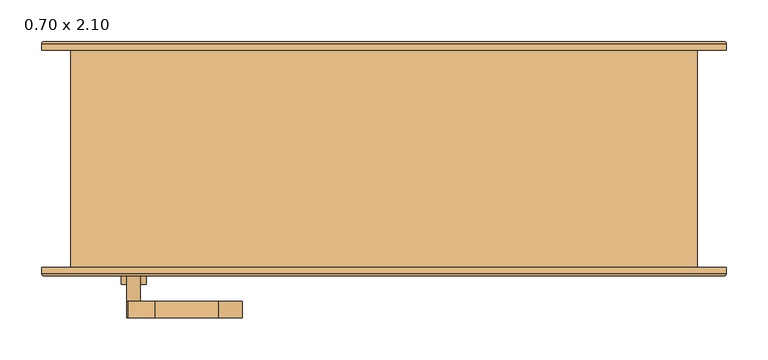
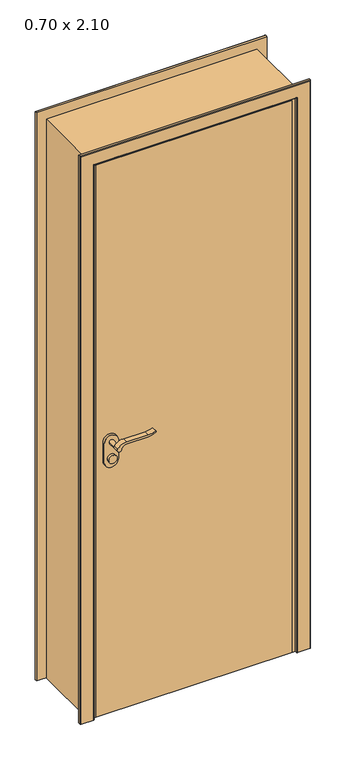
"""IFC4 building model written with IfcOpenShell, lengths in millimetres: door geometry, .CC_ND 300_PORTA SIMPLES DE ABRIR_COM EXTENSÃO : 0.70 x 2.10."""

from ifc_helpers import new_model, si_unit, point, frame, frame_2d, origin, origin_with_axes, place, context, project, spatial, polyline, circle_curve, ellipse_curve, trimmed, segment, composite_curve, outline, extrude, faceted_brep, source, transform, mapped, element, save
from ifc_brep_helpers import plane_surface, cylinder_surface, advanced_brep


def door_0_70_x_2_10_365ff999(model_context):
    return source(origin(), model_context, "Body", "SolidModel", [
        extrude(outline(composite_curve([segment(trimmed(circle_curve(frame_2d((964.5, -300.0)), 15.0), [point((964.5, -285.0))], [point((964.5, -315.0))], False, "CARTESIAN"), True, "CONTINUOUS"), segment(trimmed(circle_curve(frame_2d((964.5, -300.0)), 15.0), [point((964.5, -315.0))], [point((964.5, -285.0))], False, "CARTESIAN"), True, "CONTINUOUS")], self_intersect=False)), frame((0.0, -163.0, 0.0), z_axis=(0.0, 1.0, 0.0), x_axis=(0.0, 0.0, 1.0)), (0.0, 0.0, 1.0), 10.0),
        extrude(outline(composite_curve([segment(trimmed(circle_curve(frame_2d((964.5, -300.0)), 15.0), [point((964.5, -285.0))], [point((964.5, -315.0))], False, "CARTESIAN"), True, "CONTINUOUS"), segment(trimmed(circle_curve(frame_2d((964.5, -300.0)), 15.0), [point((964.5, -315.0))], [point((964.5, -285.0))], False, "CARTESIAN"), True, "CONTINUOUS")], self_intersect=False)), frame((0.0, -103.0, 0.0), z_axis=(0.0, 1.0, 0.0), x_axis=(0.0, 0.0, 1.0)), (0.0, 0.0, 1.0), 10.0),
        extrude(outline(composite_curve([segment(trimmed(circle_curve(frame_2d((1024.5, -300.0)), 8.0), [point((1029.1523287, -306.5081363))], [point((1024.5, -292.0))], False, "CARTESIAN"), True, "CONTINUOUS"), segment(trimmed(circle_curve(frame_2d((1019.3738613, -274.6138099)), 18.1261387), [point((1024.5, -292.0))], [point((1037.5, -274.6138099))], True, "CARTESIAN"), True, "CONTINUOUS"), segment(polyline([(1037.5, -274.6138099), (1037.5, -198.3564091)]), True, "CONTINUOUS"), segment(trimmed(circle_curve(frame_2d((1096.7709207, -201.9396612)), 59.3791355), [point((1037.5, -198.3564091))], [point((1046.7135558, -170.0))], False, "CARTESIAN"), True, "CONTINUOUS"), segment(polyline([(1046.7135558, -170.0), (1049.5, -170.0)]), True, "CONTINUOUS"), segment(trimmed(circle_curve(frame_2d((1127.7850638, -198.4227909)), 83.2850902), [point((1049.5, -170.0))], [point((1044.5, -198.3564091))], True, "CARTESIAN"), True, "CONTINUOUS"), segment(polyline([(1044.5, -198.3564091), (1044.5, -274.6325667)]), True, "CONTINUOUS"), segment(trimmed(circle_curve(frame_2d((1007.2555521, -276.3324871)), 37.2832219), [point((1044.5, -274.6325667))], [point((1029.1523287, -306.5081363))], False, "CARTESIAN"), True, "CONTINUOUS")], self_intersect=False)), frame((0.0, -203.0, 0.0), z_axis=(0.0, 1.0, 0.0), x_axis=(0.0, 0.0, 1.0)), (0.0, 0.0, 1.0), 20.0),
        extrude(outline(composite_curve([segment(trimmed(circle_curve(frame_2d((1019.3738682, -274.6138122)), 18.1261318), [point((1024.4999903, -292.0))], [point((1037.5, -274.6138122))], True, "CARTESIAN"), True, "CONTINUOUS"), segment(polyline([(1037.5, -274.6138122), (1037.5, -198.3564091)]), True, "CONTINUOUS"), segment(trimmed(circle_curve(frame_2d((1096.7709207, -201.9396612)), 59.3791355), [point((1037.5, -198.3564091))], [point((1046.7135558, -170.0))], False, "CARTESIAN"), True, "CONTINUOUS"), segment(polyline([(1046.7135558, -170.0), (1049.5, -170.0)]), True, "CONTINUOUS"), segment(trimmed(circle_curve(frame_2d((1127.7850638, -198.4227909)), 83.2850902), [point((1049.5, -170.0))], [point((1044.5, -198.3564091))], True, "CARTESIAN"), True, "CONTINUOUS"), segment(polyline([(1044.5, -198.3564091), (1044.5, -274.6325667)]), True, "CONTINUOUS"), segment(trimmed(circle_curve(frame_2d((1007.2555521, -276.3324871)), 37.2832219), [point((1044.5, -274.6325667))], [point((1029.1523287, -306.5081363))], False, "CARTESIAN"), True, "CONTINUOUS"), segment(trimmed(circle_curve(frame_2d((1024.5, -300.0)), 8.0), [point((1029.1523287, -306.5081363))], [point((1024.4999903, -292.0))], False, "CARTESIAN"), True, "CONTINUOUS")], self_intersect=False)), frame((0.0, -73.0, 0.0), z_axis=(0.0, 1.0, 0.0), x_axis=(0.0, 0.0, 1.0)), (0.0, 0.0, 1.0), 20.0),
        extrude(outline(composite_curve([segment(trimmed(circle_curve(frame_2d((1024.5, -300.0)), 8.0), [point((1024.5, -292.0))], [point((1024.5, -308.0))], False, "CARTESIAN"), True, "CONTINUOUS"), segment(trimmed(circle_curve(frame_2d((1024.5, -300.0)), 8.0), [point((1024.5, -308.0))], [point((1024.5, -292.0))], False, "CARTESIAN"), True, "CONTINUOUS")], self_intersect=False)), frame((0.0, -183.0, 0.0), z_axis=(0.0, 1.0, 0.0), x_axis=(0.0, 0.0, 1.0)), (0.0, 0.0, 1.0), 30.0),
        extrude(outline(composite_curve([segment(trimmed(circle_curve(frame_2d((1024.5, -300.0)), 8.0), [point((1024.5, -292.0))], [point((1024.5, -308.0))], False, "CARTESIAN"), True, "CONTINUOUS"), segment(trimmed(circle_curve(frame_2d((1024.5, -300.0)), 8.0), [point((1024.5, -308.0))], [point((1024.5, -292.0))], False, "CARTESIAN"), True, "CONTINUOUS")], self_intersect=False)), frame((0.0, -103.0, 0.0), z_axis=(0.0, 1.0, 0.0), x_axis=(0.0, 0.0, 1.0)), (0.0, 0.0, 1.0), 30.0),
        extrude(outline(composite_curve([segment(trimmed(circle_curve(frame_2d((954.5, -300.0)), 25.0), [point((954.5, -325.0))], [point((954.5, -275.0))], False, "CARTESIAN"), True, "CONTINUOUS"), segment(polyline([(954.5, -275.0), (1024.5, -275.0)]), True, "CONTINUOUS"), segment(trimmed(circle_curve(frame_2d((1024.5, -300.0)), 25.0), [point((1024.5, -275.0))], [point((1024.5, -325.0))], False, "CARTESIAN"), True, "CONTINUOUS"), segment(polyline([(1024.5, -325.0), (954.5, -325.0)]), True, "CONTINUOUS")], self_intersect=False)), frame((0.0, -153.0, 0.0), z_axis=(0.0, 1.0, 0.0), x_axis=(0.0, 0.0, 1.0)), (0.0, 0.0, 1.0), 10.0),
        extrude(outline(composite_curve([segment(trimmed(circle_curve(frame_2d((954.5, -300.0)), 25.0), [point((954.5, -325.0))], [point((954.5, -275.0))], False, "CARTESIAN"), True, "CONTINUOUS"), segment(polyline([(954.5, -275.0), (1024.5, -275.0)]), True, "CONTINUOUS"), segment(trimmed(circle_curve(frame_2d((1024.5, -300.0)), 25.0), [point((1024.5, -275.0))], [point((1024.5, -325.0))], False, "CARTESIAN"), True, "CONTINUOUS"), segment(polyline([(1024.5, -325.0), (954.5, -325.0)]), True, "CONTINUOUS")], self_intersect=False)), frame((0.0, -113.0, 0.0), z_axis=(0.0, 1.0, 0.0), x_axis=(0.0, 0.0, 1.0)), (0.0, 0.0, 1.0), 10.0),
        advanced_brep(
        [(-410.0, -143.0, 0.0), (-360.0, -143.0, 0.0), (-360.0, -150.0, 0.0), (-363.0, -153.0, 0.0), (-407.0, -153.0, 0.0), (-410.0, -150.0, 0.0), (-410.0, -143.0, 2135.0), (410.0, -143.0, 2135.0), (410.0, -143.0, 0.0), (360.0, -143.0, 0.0), (360.0, -143.0, 2085.0), (-360.0, -143.0, 2085.0), (-360.0, -150.0, 2085.0), (-363.0, -153.0, 2088.0), (363.0, -153.0, 2088.0), (363.0, -153.0, 0.0), (407.0, -153.0, 0.0), (407.0, -153.0, 2132.0), (-407.0, -153.0, 2132.0), (-410.0, -150.0, 2135.0), (410.0, -150.0, 2135.0), (410.0, -150.0, 0.0), (360.0, -150.0, 0.0), (360.0, -150.0, 2085.0)],
        [
            (0, 1),
            (1, 2),
            (2, 3, circle_curve(frame((-363.0, -150.0, 0.0), z_axis=(0.0, 0.0, -1.0), x_axis=(1.0, 0.0, 0.0)), 3.0)),
            (3, 4),
            (4, 5, circle_curve(frame((-407.0, -150.0, 0.0), z_axis=(0.0, 0.0, -1.0), x_axis=(1.0, 0.0, 0.0)), 3.0)),
            (5, 0),
            (0, 6),
            (6, 7),
            (7, 8),
            (8, 9),
            (9, 10),
            (10, 11),
            (11, 1),
            (11, 12),
            (12, 2),
            (12, 13, ellipse_curve(frame((-363.0, -150.0, 2088.0), z_axis=(-0.7071067811865475, 0.0, -0.7071067811865475), x_axis=(0.7071067811865474, 0.0, -0.7071067811865476)), 4.2426407, 3.0)),
            (13, 3),
            (13, 14),
            (14, 15),
            (15, 16),
            (16, 17),
            (17, 18),
            (18, 4),
            (18, 19, ellipse_curve(frame((-407.0, -150.0, 2132.0), z_axis=(-0.7071067811865475, 0.0, -0.7071067811865475), x_axis=(0.7071067811865474, 0.0, -0.7071067811865476)), 4.2426407, 3.0)),
            (19, 5),
            (19, 6),
            (7, 20),
            (20, 21),
            (21, 8),
            (21, 16, circle_curve(frame((407.0, -150.0, 0.0), z_axis=(0.0, 0.0, -1.0), x_axis=(-1.0, 0.0, 0.0)), 3.0)),
            (15, 22, circle_curve(frame((363.0, -150.0, 0.0), z_axis=(0.0, 0.0, -1.0), x_axis=(-1.0, 0.0, 0.0)), 3.0)),
            (22, 9),
            (23, 10),
            (22, 23),
            (14, 23, ellipse_curve(frame((363.0, -150.0, 2088.0), z_axis=(0.7071067811865475, 0.0, -0.7071067811865475), x_axis=(0.7071067811865474, 0.0, 0.7071067811865476)), 4.2426407, 3.0)),
            (20, 17, ellipse_curve(frame((407.0, -150.0, 2132.0), z_axis=(0.7071067811865475, 0.0, -0.7071067811865475), x_axis=(0.7071067811865474, 0.0, 0.7071067811865476)), 4.2426407, 3.0)),
            (23, 12),
            (19, 20),
        ],
        [
            plane_surface(frame((-360.0, -143.0, 0.0), z_axis=(0.0, 0.0, -1.0), x_axis=(0.0, 1.0, 0.0))),
            plane_surface(frame((-410.0, -143.0, 0.0), z_axis=(0.0, 1.0, 0.0), x_axis=(0.0, 0.0, 1.0))),
            plane_surface(frame((-360.0, -143.0, 0.0), z_axis=(1.0, 0.0, 0.0), x_axis=(0.0, 0.0, 1.0))),
            cylinder_surface(frame((-363.0, -150.0, 0.0), z_axis=(0.0, 0.0, -1.0), x_axis=(1.0, 0.0, 0.0)), 3.0),
            plane_surface(frame((-363.0, -153.0, 0.0), z_axis=(0.0, -1.0, 0.0), x_axis=(0.0, 0.0, 1.0))),
            cylinder_surface(frame((-407.0, -150.0, 0.0), z_axis=(0.0, 0.0, -1.0), x_axis=(1.0, 0.0, 0.0)), 3.0),
            plane_surface(frame((-410.0, -150.0, 0.0), z_axis=(-1.0, 0.0, 0.0), x_axis=(0.0, 0.0, 1.0))),
            plane_surface(frame((410.0, -150.0, 2135.0), z_axis=(1.0, 0.0, 0.0), x_axis=(0.0, 0.0, -1.0))),
            plane_surface(frame((360.0, -143.0, 0.0), z_axis=(0.0, 0.0, -1.0), x_axis=(0.0, 1.0, 0.0))),
            plane_surface(frame((360.0, -143.0, 2085.0), z_axis=(-1.0, 0.0, 0.0), x_axis=(0.0, 0.0, -1.0))),
            cylinder_surface(frame((363.0, -150.0, 2085.0), z_axis=(0.0, 0.0, 1.0), x_axis=(-1.0, 0.0, 0.0)), 3.0),
            cylinder_surface(frame((407.0, -150.0, 2085.0), z_axis=(0.0, 0.0, 1.0), x_axis=(-1.0, 0.0, 0.0)), 3.0),
            plane_surface(frame((-360.0, -143.0, 2085.0), z_axis=(0.0, 0.0, -1.0), x_axis=(1.0, 0.0, 0.0))),
            plane_surface(frame((-410.0, -150.0, 2135.0), z_axis=(0.0, 0.0, 1.0), x_axis=(1.0, 0.0, 0.0))),
            cylinder_surface(frame((-360.0, -150.0, 2088.0), z_axis=(-1.0, 0.0, 0.0), x_axis=(0.0, 0.0, -1.0)), 3.0),
            cylinder_surface(frame((-360.0, -150.0, 2132.0), z_axis=(-1.0, 0.0, 0.0), x_axis=(0.0, 0.0, -1.0)), 3.0),
        ],
        [
            (0, [[1, 2, 3, 4, 5, 6]]),
            (1, [[-1, 7, 8, 9, 10, 11, 12, 13]]),
            (2, [[-2, -13, 14, 15]]),
            (3, [[-3, -15, 16, 17]]),
            (4, [[-4, -17, 18, 19, 20, 21, 22, 23]]),
            (5, [[-5, -23, 24, 25]]),
            (6, [[-6, -25, 26, -7]]),
            (7, [[27, 28, 29, -9]]),
            (8, [[-29, 30, -20, 31, 32, -10]]),
            (9, [[33, -11, -32, 34]]),
            (10, [[35, -34, -31, -19]]),
            (11, [[36, -21, -30, -28]]),
            (12, [[-14, -12, -33, 37]]),
            (13, [[-26, 38, -27, -8]]),
            (14, [[-16, -37, -35, -18]]),
            (15, [[-24, -22, -36, -38]]),
        ],
    ),
        advanced_brep(
        [(410.0, 118.0, 0.0), (360.0, 118.0, 0.0), (360.0, 125.0157283, 0.0), (362.9842717, 128.0, 0.0), (407.0342217, 128.0, 0.0), (410.0, 125.0342217, 0.0), (410.0, 118.0, 2135.0), (-410.0, 118.0, 2135.0), (-410.0, 118.0, 0.0), (-360.0, 118.0, 0.0), (-360.0, 118.0, 2085.0), (360.0, 118.0, 2085.0), (360.0, 125.0157283, 2085.0), (362.9842717, 128.0, 2087.9842717), (-362.9842717, 128.0, 2087.9842717), (-362.9842717, 128.0, 0.0), (-407.0342217, 128.0, 0.0), (-407.0342217, 128.0, 2132.0342217), (407.0342217, 128.0, 2132.0342217), (410.0, 125.0342217, 2135.0), (-410.0, 125.0342217, 2135.0), (-410.0, 125.0342217, 0.0), (-360.0, 125.0157283, 0.0), (-360.0, 125.0157283, 2085.0)],
        [
            (0, 1),
            (1, 2),
            (2, 3, circle_curve(frame((362.9842717, 125.0157283, 0.0), z_axis=(0.0, 0.0, -1.0), x_axis=(1.0, 0.0, 0.0)), 2.9842717)),
            (3, 4),
            (4, 5, circle_curve(frame((407.0342217, 125.0342217, 0.0), z_axis=(0.0, 0.0, -1.0), x_axis=(1.0, 0.0, 0.0)), 2.9657783)),
            (5, 0),
            (0, 6),
            (6, 7),
            (7, 8),
            (8, 9),
            (9, 10),
            (10, 11),
            (11, 1),
            (11, 12),
            (12, 2),
            (12, 13, ellipse_curve(frame((362.9842717, 125.0157283, 2087.9842717), z_axis=(0.7071067811865475, 0.0, -0.7071067811865475), x_axis=(-0.7071067811865474, 0.0, -0.7071067811865476)), 4.2203975, 2.9842717)),
            (13, 3),
            (13, 14),
            (14, 15),
            (15, 16),
            (16, 17),
            (17, 18),
            (18, 4),
            (18, 19, ellipse_curve(frame((407.0342217, 125.0342217, 2132.0342217), z_axis=(0.7071067811865475, 0.0, -0.7071067811865475), x_axis=(-0.7071067811865474, 0.0, -0.7071067811865476)), 4.1942438, 2.9657783)),
            (19, 5),
            (19, 6),
            (7, 20),
            (20, 21),
            (21, 8),
            (21, 16, circle_curve(frame((-407.0342217, 125.0342217, 0.0), z_axis=(0.0, 0.0, -1.0), x_axis=(-1.0, 0.0, 0.0)), 2.9657783)),
            (15, 22, circle_curve(frame((-362.9842717, 125.0157283, 0.0), z_axis=(0.0, 0.0, -1.0), x_axis=(-1.0, 0.0, 0.0)), 2.9842717)),
            (22, 9),
            (23, 10),
            (22, 23),
            (14, 23, ellipse_curve(frame((-362.9842717, 125.0157283, 2087.9842717), z_axis=(-0.7071067811865475, 0.0, -0.7071067811865475), x_axis=(-0.7071067811865474, 0.0, 0.7071067811865476)), 4.2203975, 2.9842717)),
            (20, 17, ellipse_curve(frame((-407.0342217, 125.0342217, 2132.0342217), z_axis=(-0.7071067811865475, 0.0, -0.7071067811865475), x_axis=(-0.7071067811865474, 0.0, 0.7071067811865476)), 4.1942438, 2.9657783)),
            (23, 12),
            (19, 20),
        ],
        [
            plane_surface(frame((360.0, 118.0, 0.0), z_axis=(0.0, 0.0, -1.0), x_axis=(0.0, 1.0, 0.0))),
            plane_surface(frame((410.0, 118.0, 0.0), z_axis=(0.0, -1.0, 0.0), x_axis=(0.0, 0.0, 1.0))),
            plane_surface(frame((360.0, 118.0, 0.0), z_axis=(-1.0, 0.0, 0.0), x_axis=(0.0, 0.0, 1.0))),
            cylinder_surface(frame((362.9842717, 125.0157283, 0.0), z_axis=(0.0, 0.0, -1.0), x_axis=(1.0, 0.0, 0.0)), 2.9842717),
            plane_surface(frame((362.9842717, 128.0, 0.0), z_axis=(0.0, 1.0, 0.0), x_axis=(0.0, 0.0, 1.0))),
            cylinder_surface(frame((407.0342217, 125.0342217, 0.0), z_axis=(0.0, 0.0, -1.0), x_axis=(1.0, 0.0, 0.0)), 2.9657783),
            plane_surface(frame((410.0, 125.0342217, 0.0), z_axis=(1.0, 0.0, 0.0), x_axis=(0.0, 0.0, 1.0))),
            plane_surface(frame((-410.0, 125.0342217, 2135.0), z_axis=(-1.0, 0.0, 0.0), x_axis=(0.0, 0.0, -1.0))),
            plane_surface(frame((-360.0, 118.0, 0.0), z_axis=(0.0, 0.0, -1.0), x_axis=(0.0, 1.0, 0.0))),
            plane_surface(frame((-360.0, 118.0, 2085.0), z_axis=(1.0, 0.0, 0.0), x_axis=(0.0, 0.0, -1.0))),
            cylinder_surface(frame((-362.9842717, 125.0157283, 2085.0), z_axis=(0.0, 0.0, 1.0), x_axis=(-1.0, 0.0, 0.0)), 2.9842717),
            cylinder_surface(frame((-407.0342217, 125.0342217, 2085.0), z_axis=(0.0, 0.0, 1.0), x_axis=(-1.0, 0.0, 0.0)), 2.9657783),
            plane_surface(frame((360.0, 118.0, 2085.0), z_axis=(0.0, 0.0, -1.0), x_axis=(-1.0, 0.0, 0.0))),
            plane_surface(frame((410.0, 125.0342217, 2135.0), z_axis=(0.0, 0.0, 1.0), x_axis=(-1.0, 0.0, 0.0))),
            cylinder_surface(frame((360.0, 125.0157283, 2087.9842717), z_axis=(1.0, 0.0, 0.0), x_axis=(0.0, 0.0, 1.0)), 2.9842717),
            cylinder_surface(frame((360.0, 125.0342217, 2132.0342217), z_axis=(1.0, 0.0, 0.0), x_axis=(0.0, 0.0, 1.0)), 2.9657783),
        ],
        [
            (0, [[1, 2, 3, 4, 5, 6]]),
            (1, [[-1, 7, 8, 9, 10, 11, 12, 13]]),
            (2, [[-2, -13, 14, 15]]),
            (3, [[-3, -15, 16, 17]]),
            (4, [[-4, -17, 18, 19, 20, 21, 22, 23]]),
            (5, [[-5, -23, 24, 25]]),
            (6, [[-6, -25, 26, -7]]),
            (7, [[27, 28, 29, -9]]),
            (8, [[-29, 30, -20, 31, 32, -10]]),
            (9, [[33, -11, -32, 34]]),
            (10, [[35, -34, -31, -19]]),
            (11, [[36, -21, -30, -28]]),
            (12, [[-14, -12, -33, 37]]),
            (13, [[-26, 38, -27, -8]]),
            (14, [[-16, -37, -35, -18]]),
            (15, [[-24, -22, -36, -38]]),
        ],
    ),
        faceted_brep([(342.0, 118.0, 0.0), (375.0, 118.0, 0.0), (375.0, -143.0, 0.0), (350.0, -143.0, 0.0), (350.0, -113.0, 0.0), (342.0, -113.0, 0.0), (342.0, 118.0, 2067.0), (-342.0, 118.0, 2067.0), (-342.0, 118.0, 0.0), (-375.0, 118.0, 0.0), (-375.0, 118.0, 2100.0), (375.0, 118.0, 2100.0), (375.0, -143.0, 2100.0), (-375.0, -143.0, 2100.0), (-375.0, -143.0, 0.0), (-350.0, -143.0, 0.0), (-350.0, -143.0, 2075.0), (350.0, -143.0, 2075.0), (350.0, -113.0, 2075.0), (-350.0, -113.0, 2075.0), (-350.0, -113.0, 0.0), (-342.0, -113.0, 0.0), (-342.0, -113.0, 2067.0), (342.0, -113.0, 2067.0)], [[[0, 1, 2, 3, 4, 5]], [[1, 0, 6, 7, 8, 9, 10, 11]], [[2, 1, 11, 12]], [[3, 2, 12, 13, 14, 15, 16, 17]], [[4, 3, 17, 18]], [[5, 4, 18, 19, 20, 21, 22, 23]], [[0, 5, 23, 6]], [[7, 22, 21, 8]], [[8, 21, 20, 15, 14, 9]], [[13, 10, 9, 14]], [[19, 16, 15, 20]], [[12, 11, 10, 13]], [[18, 17, 16, 19]], [[6, 23, 22, 7]]]),
        extrude(outline(polyline([(-350.0, -113.0), (350.0, -113.0), (350.0, -143.0), (-350.0, -143.0), (-350.0, -113.0)])), origin_with_axes(), (0.0, 0.0, 1.0), 2075.0),
    ])


if __name__ == "__main__":
    model = new_model("IFC4")
    model_context = context("Model", 3, world=origin())
    ifc_project = project(units=[si_unit("LENGTHUNIT", "METRE", prefix="MILLI")], contexts=[model_context])
    site = spatial("IfcSite", under=ifc_project)
    building = spatial("IfcBuilding", under=site)
    placement = place(None, origin())
    door_0_70_x_2_10_shape = door_0_70_x_2_10_365ff999(model_context)
    element("IfcDoor", 1, ObjectType=".CC_ND 300_PORTA SIMPLES DE ABRIR_COM EXTENSÃO : 0.70 x 2.10", at=placement, inside=building, context=model_context, shape_type="MappedRepresentation", body=[
        mapped(door_0_70_x_2_10_shape, transform((0.0, 0.0, 0.0), x_axis=(1.0, 0.0, 0.0), y_axis=(0.0, 1.0, 0.0), z_axis=(0.0, 0.0, 1.0))),
    ])
    save(model, "model.ifc")

# Revit data of these elements
# Type ".CC_ND 300_PORTA SIMPLES DE ABRIR_COM EXTENSÃO : 0.70 x 2.10"
#   Type Mark = "155"
#   Rough Width = 0.75 m
#   Espessura moldura externa = 0.01 m
#   Espessura moldura interna = 0.01 m
#   Largura moldura = 0.05 m
#   Extensão acabamento exterior [instance default] = 0.00 m
#   Extensão acabamento interior [instance default] = 0.00 m
#   Espessura batente = 0.025 m
#   Thickness = 0.03 m
#   Altura batente = 2.085 m
#   Aux Arco [instance default] = 0.70 m
#   Rough Height = 2.125 m
#   Height = 2.10 m
#   Width = 0.70 m
#   Moldura interna [instance default] = yes
#   Moldura externa [instance default] = yes
#   Porta = .MADEIRA COM PINTURA ESMALTE BRANCO ACETINADO
#   Moldura = .MADEIRA COM PINTURA ESMALTE BRANCO ACETINADO
#   Maçaneta = .ALUMÍNIO
#   Batente = .MADEIRA COM PINTURA ESMALTE BRANCO ACETINADO
#   Function = (empty or 0)
#   Wall Closure = (empty or 0)
# Element 1 (IfcDoor, ".CC_ND 300_PORTA SIMPLES DE ABRIR_COM EXTENSÃO : 0.70 x 2.10")
#   Extensão acabamento interior = 0.025 m
#   Aux Arco = 0.725 m
#   Materials on its faces: ".MADEIRA COM PINTURA ESMALTE BRANCO ACETINADO", ".ALUMÍNIO"
# Materials
#   ".MADEIRA COM PINTURA ESMALTE BRANCO ACETINADO": class ".CC_MADEIRAS", colour RGB 240 240 240, transparency 0, Description = "Madeira com pintura esmalte branco acetinado.", Cost = 0
#   ".ALUMÍNIO": class "CC_METAIS", colour RGB 244 244 244, transparency 0, Description = "Material alumínio", Cost = 0
